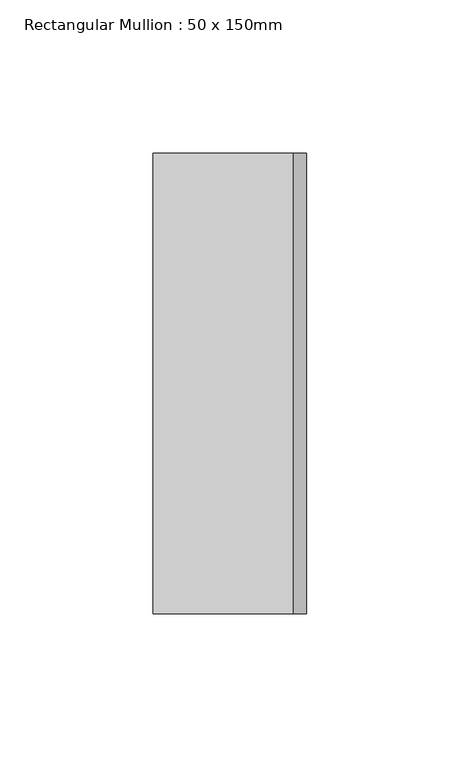
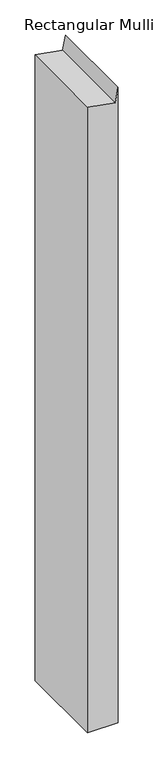
"""IFC4 building model written with IfcOpenShell, lengths in millimetres: member geometry, Rectangular Mullion : 50 x 150mm."""

from ifc_helpers import new_model, si_unit, frame, origin, place, context, project, spatial, polyline, outline, extrude, source, transform, mapped, element, save


def rectangular_mullion_50_x_150mm_e8a3ed51(model_context):
    return source(origin(), model_context, "Body", "SweptSolid", [
        extrude(outline(polyline([(25.0, 0.0), (0.3798062, -4.3412044), (8.4306837, -50.0), (-1078.6304927, -50.0), (-1078.6304927, 0.0), (25.0, 0.0)])), frame((0.0, -75.0, 0.0), z_axis=(0.0, 1.0, 0.0), x_axis=(0.0, 0.0, 1.0)), (0.0, 0.0, 1.0), 150.0),
    ])


if __name__ == "__main__":
    model = new_model("IFC4")
    model_context = context("Model", 3, world=origin())
    ifc_project = project(units=[si_unit("LENGTHUNIT", "METRE", prefix="MILLI")], contexts=[model_context])
    site = spatial("IfcSite", under=ifc_project)
    building = spatial("IfcBuilding", under=site)
    placement = place(None, origin())
    rectangular_mullion_50_x_150mm_shape = rectangular_mullion_50_x_150mm_e8a3ed51(model_context)
    element("IfcMember", 1, ObjectType="Rectangular Mullion : 50 x 150mm", at=placement, inside=building, context=model_context, shape_type="MappedRepresentation", body=[
        mapped(rectangular_mullion_50_x_150mm_shape, transform((0.0, 0.0, 0.0), x_axis=(1.0, 0.0, 0.0), y_axis=(0.0, 1.0, 0.0), z_axis=(0.0, 0.0, 1.0))),
    ])
    save(model, "model.ifc")

# Revit data of these elements
# Type "Rectangular Mullion : 50 x 150mm"
#   built-in parameter 1007304 = 0.492126 (stored number, unit not read)
#   built-in parameter 1007301 = 0.082021 (stored number, unit not read)
#   built-in parameter 1007300 = 0.082021 (stored number, unit not read)
# Element 1 (IfcMember, "Rectangular Mullion : 50 x 150mm")
#   Materials on its faces: "Aluminium"
# Materials
#   "Aluminium": class "Metal", colour RGB 247 247 247, transparency 0, Description = "Aluminium 6061", Cost = 0
